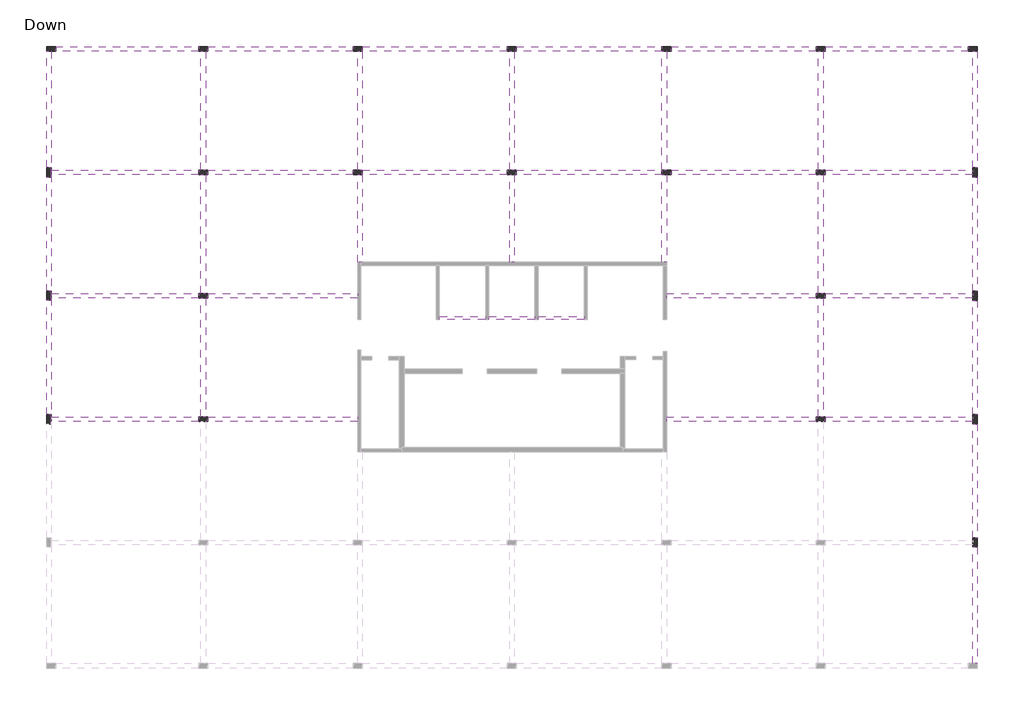
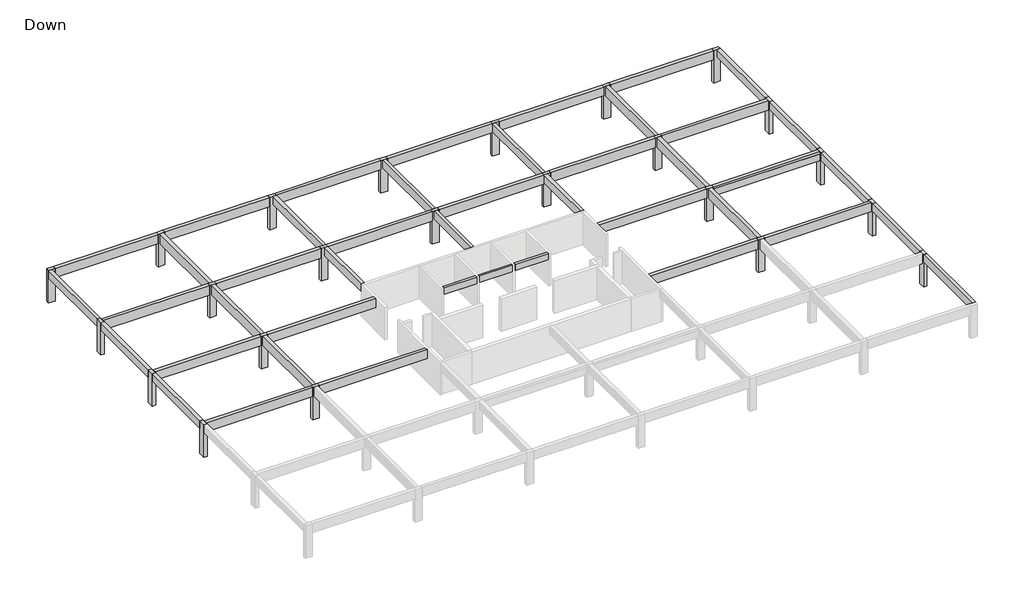
# One storey, part 2 of 2: 43 beams, 23 columns.
"""IFC4 building model written with IfcOpenShell, lengths in millimetres."""

from ifc_helpers import new_model, si_unit, frame, origin, origin_with_axes, place, context, project, spatial, polyline, outline, extrude, faceted_brep, element, save

model = new_model("IFC4")

# Units and contexts
model_context = context("Model", 3, world=origin())
ifc_project = project(units=[si_unit("LENGTHUNIT", "METRE", prefix="MILLI")], contexts=[model_context])

# Site, building, storey
site = spatial("IfcSite", under=ifc_project)
building = spatial("IfcBuilding", under=site)
storey = spatial("IfcBuildingStorey", under=building, Name="Down", Elevation=0.0)

# Beams
placement = place(None, origin())
element("IfcBeam", 1, ObjectType="Concrete Rectengular Beam : 20/60", at=placement, inside=storey, context=model_context, shape_type="SweptSolid", body=[
    extrude(outline(polyline([(-1146.9159577, 7369.5351037), (-1146.9159577, 7569.5351037), (1839.2018335, 7569.5351037), (1839.2018335, 7369.5351037), (-1146.9159577, 7369.5351037)])), frame((0.0, 0.0, 2480.0), z_axis=(0.0, 0.0, 1.0), x_axis=(1.0, 0.0, 0.0)), (0.0, 0.0, 1.0), 600.0),
])
element("IfcBeam", 2, ObjectType="Concrete Rectengular Beam : 20/60", at=placement, inside=storey, context=model_context, shape_type="Brep", body=[
    faceted_brep([(2039.2018335, 7569.5351037, 3080.0), (2039.2018335, 7369.5351037, 3080.0), (5039.2018335, 7369.5351037, 3080.0), (5039.2018335, 7569.5351037, 3080.0), (2039.2018335, 7369.5351037, 2860.0), (2039.2018335, 7369.5351037, 2480.0), (5039.2018335, 7369.5351037, 2480.0), (2039.2018335, 7569.5351037, 2480.0), (5039.2018335, 7569.5351037, 2480.0)], [[[0, 1, 2, 3]], [[1, 4, 5, 6, 2]], [[5, 7, 8, 6]], [[7, 0, 3, 8]], [[1, 0, 7, 5, 4]], [[3, 2, 6, 8]]]),
])
element("IfcBeam", 3, ObjectType="Concrete Rectengular Beam : 20/60", at=placement, inside=storey, context=model_context, shape_type="Brep", body=[
    faceted_brep([(5239.2018335, 7569.5351037, 3080.0), (5239.2018335, 7369.5351037, 3080.0), (8239.2018335, 7369.5351037, 3080.0), (8239.2018335, 7569.5351037, 3080.0), (5239.2018335, 7369.5351037, 2860.0), (5239.2018335, 7369.5351037, 2480.0), (8239.2018335, 7369.5351037, 2480.0), (5239.2018335, 7569.5351037, 2480.0), (8239.2018335, 7569.5351037, 2480.0)], [[[0, 1, 2, 3]], [[1, 4, 5, 6, 2]], [[5, 7, 8, 6]], [[7, 0, 3, 8]], [[1, 0, 7, 5, 4]], [[3, 2, 6, 8]]]),
])
element("IfcBeam", 4, ObjectType="Concrete Rectengular Beam : 30/70", at=placement, inside=storey, context=model_context, shape_type="SweptSolid", body=[
    extrude(outline(polyline([(33698.6447783, 9222.0890048), (33398.6447783, 9222.0890048), (33398.6447783, 16622.0890048), (33698.6447783, 16622.0890048), (33698.6447783, 9222.0890048)])), frame((0.0, 0.0, 2380.0), z_axis=(0.0, 0.0, 1.0), x_axis=(1.0, 0.0, 0.0)), (0.0, 0.0, 1.0), 700.0),
])
element("IfcBeam", 5, ObjectType="Concrete Rectengular Beam : 30/70", at=placement, inside=storey, context=model_context, shape_type="SweptSolid", body=[
    extrude(outline(polyline([(33398.6447783, 8622.0890048), (33698.6447783, 8622.0890048), (33698.6447783, 1224.102585), (33398.6447783, 1224.102585), (33398.6447783, 8622.0890048)])), frame((0.0, 0.0, 2380.0), z_axis=(0.0, 0.0, 1.0), x_axis=(1.0, 0.0, 0.0)), (0.0, 0.0, 1.0), 700.0),
])
element("IfcBeam", 6, ObjectType="Concrete Rectengular Beam : 30/70", at=placement, inside=storey, context=model_context, shape_type="SweptSolid", body=[
    extrude(outline(polyline([(33698.6447783, -6770.4648963), (33398.6447783, -6770.4648963), (33398.6447783, 624.102585), (33698.6447783, 624.102585), (33698.6447783, -6770.4648963)])), frame((0.0, 0.0, 2380.0), z_axis=(0.0, 0.0, 1.0), x_axis=(1.0, 0.0, 0.0)), (0.0, 0.0, 1.0), 700.0),
])
element("IfcBeam", 7, ObjectType="Concrete Rectengular Beam : 30/70", at=placement, inside=storey, context=model_context, shape_type="Brep", body=[
    faceted_brep([(33698.6447783, -7370.4648963, 3080.0), (33398.6447783, -7370.4648963, 3080.0), (33398.6447783, -14918.7716477, 3080.0), (33698.6447783, -14918.7716477, 3080.0), (33398.6447783, -7370.4648963, 2380.0), (33398.6447783, -14918.7716477, 2380.0), (33398.6447783, -14918.7716477, 2860.0), (33698.6447783, -7370.4648963, 2380.0), (33698.6447783, -14918.7716477, 2380.0)], [[[0, 1, 2, 3]], [[1, 4, 5, 6, 2]], [[4, 7, 8, 5]], [[7, 0, 3, 8]], [[1, 0, 7, 4]], [[3, 2, 6, 5, 8]]]),
])
element("IfcBeam", 8, ObjectType="Concrete Rectengular Beam : 30/70", at=placement, inside=storey, context=model_context, shape_type="Brep", body=[
    faceted_brep([(33698.6447783, 24775.4190544, 3080.0), (33398.6447783, 24775.4190544, 3080.0), (33398.6447783, 17222.0890048, 3080.0), (33698.6447783, 17222.0890048, 3080.0), (33398.6447783, 24775.4190544, 2860.0), (33398.6447783, 24775.4190544, 2380.0), (33398.6447783, 17222.0890048, 2380.0), (33698.6447783, 24775.4190544, 2380.0), (33698.6447783, 17222.0890048, 2380.0)], [[[0, 1, 2, 3]], [[1, 4, 5, 6, 2]], [[5, 7, 8, 6]], [[7, 0, 3, 8]], [[1, 0, 7, 5, 4]], [[3, 2, 6, 8]]]),
])
element("IfcBeam", 9, ObjectType="Concrete Rectengular Beam : 30/70", at=placement, inside=storey, context=model_context, shape_type="Brep", body=[
    faceted_brep([(-26299.591421, 9078.7943074, 3080.0), (-26299.591421, 8628.7943074, 3080.0), (-26599.1167382, 8628.7943074, 3080.0), (-26599.1167382, 1224.102585, 3080.0), (-26299.591421, 1224.102585, 3080.0), (-26299.591421, 1074.102585, 3080.0), (-26299.1167382, 1074.102585, 3080.0), (-26299.1167382, 8778.7943074, 3080.0), (-26299.1167382, 9078.7943074, 3080.0), (-26299.1167382, 9078.7943074, 2380.0), (-26299.1167382, 1074.102585, 2860.0), (-26299.1167382, 1074.102585, 2380.0), (-26299.1167382, 8778.7943074, 2380.0), (-26299.591421, 8628.7943074, 2380.0), (-26299.591421, 8778.7943074, 2380.0), (-26299.591421, 9078.7943074, 2380.0), (-26299.591421, 1074.102585, 2380.0), (-26299.591421, 1224.102585, 2380.0), (-26599.1167382, 1224.102585, 2380.0), (-26599.1167382, 8628.7943074, 2380.0)], [[[0, 1, 2, 3, 4, 5, 6, 7, 8]], [[9, 8, 7, 6, 10, 11, 12]], [[13, 14, 15, 9, 12, 11, 16, 17, 18, 19]], [[2, 19, 18, 3]], [[13, 1, 0, 15, 14]], [[1, 13, 19, 2]], [[17, 4, 3, 18]], [[4, 17, 16, 5]], [[8, 9, 15, 0]], [[11, 10, 6, 5, 16]]]),
])
element("IfcBeam", 10, ObjectType="Concrete Rectengular Beam : 30/70", at=placement, inside=storey, context=model_context, shape_type="Brep", body=[
    faceted_brep([(-26299.591421, 17073.0342824, 3080.0), (-26299.591421, 16623.0342824, 3080.0), (-26599.1167382, 16623.0342824, 3080.0), (-26599.1167382, 9228.7943074, 3080.0), (-26299.591421, 9228.7943074, 3080.0), (-26299.591421, 9078.7943074, 3080.0), (-26299.1167382, 9078.7943074, 3080.0), (-26299.1167382, 16773.0342824, 3080.0), (-26299.1167382, 17073.0342824, 3080.0), (-26299.1167382, 9078.7943074, 2860.0), (-26299.1167382, 9078.7943074, 2380.0), (-26299.1167382, 16773.0342824, 2380.0), (-26299.1167382, 17073.0342824, 2380.0), (-26299.591421, 16623.0342824, 2380.0), (-26299.591421, 16773.0342824, 2380.0), (-26299.591421, 17073.0342824, 2380.0), (-26299.591421, 9078.7943074, 2380.0), (-26299.591421, 9228.7943074, 2380.0), (-26599.1167382, 9228.7943074, 2380.0), (-26599.1167382, 16623.0342824, 2380.0)], [[[0, 1, 2, 3, 4, 5, 6, 7, 8]], [[6, 9, 10, 11, 12, 8, 7]], [[13, 14, 15, 12, 11, 10, 16, 17, 18, 19]], [[2, 19, 18, 3]], [[13, 1, 0, 15, 14]], [[1, 13, 19, 2]], [[17, 4, 3, 18]], [[4, 17, 16, 5]], [[10, 9, 6, 5, 16]], [[8, 12, 15, 0]]]),
])
element("IfcBeam", 11, ObjectType="Concrete Rectengular Beam : 30/70", at=placement, inside=storey, context=model_context, shape_type="Brep", body=[
    faceted_brep([(-26299.1167382, 24775.4190544, 3080.0), (-26599.1167382, 24775.4190544, 3080.0), (-26599.1167382, 17223.0342824, 3080.0), (-26299.591421, 17223.0342824, 3080.0), (-26299.591421, 17073.0342824, 3080.0), (-26299.1167382, 17073.0342824, 3080.0), (-26299.1167382, 24775.4190544, 2380.0), (-26299.1167382, 24775.4190544, 2860.0), (-26299.1167382, 17073.0342824, 2860.0), (-26299.1167382, 17073.0342824, 2380.0), (-26599.1167382, 24775.4190544, 2380.0), (-26299.591421, 17073.0342824, 2380.0), (-26299.591421, 17223.0342824, 2380.0), (-26599.1167382, 17223.0342824, 2380.0)], [[[0, 1, 2, 3, 4, 5]], [[6, 7, 0, 5, 8, 9]], [[10, 6, 9, 11, 12, 13]], [[1, 10, 13, 2]], [[1, 0, 7, 6, 10]], [[12, 3, 2, 13]], [[3, 12, 11, 4]], [[9, 8, 5, 4, 11]]]),
])
element("IfcBeam", 12, ObjectType="Concrete Rectengular Beam : 30/75", at=placement, inside=storey, context=model_context, shape_type="Brep", body=[
    faceted_brep([(-6447.328783, 17073.0342824, 3080.0), (-6147.328783, 17073.0342824, 3080.0), (-6147.328783, 24775.4190544, 3080.0), (-6447.328783, 24775.4190544, 3080.0), (-6447.328783, 17073.0342824, 2330.0), (-6447.328783, 17073.0342824, 2860.0), (-6447.328783, 24775.4190544, 2860.0), (-6447.328783, 24775.4190544, 2330.0), (-6147.328783, 17073.0342824, 2330.0), (-6147.328783, 24775.4190544, 2330.0), (-6147.328783, 17073.0342824, 2860.0), (-6147.328783, 24775.4190544, 2860.0)], [[[0, 1, 2, 3]], [[4, 5, 0, 3, 6, 7]], [[8, 4, 7, 9]], [[1, 10, 8, 9, 11, 2]], [[1, 0, 5, 4, 8, 10]], [[3, 2, 11, 9, 7, 6]]]),
])
element("IfcBeam", 13, ObjectType="Concrete Rectengular Beam : 30/75", at=placement, inside=storey, context=model_context, shape_type="Brep", body=[
    faceted_brep([(-6147.328783, 16773.0342824, 3080.0), (-6447.328783, 16773.0342824, 3080.0), (-6447.328783, 11089.5351037, 3080.0), (-6247.328783, 11089.5351037, 3080.0), (-6147.328783, 11089.5351037, 3080.0), (-6447.328783, 16773.0342824, 2860.0), (-6447.328783, 16773.0342824, 2330.0), (-6447.328783, 11089.5351037, 2330.0), (-6147.328783, 16773.0342824, 2330.0), (-6147.328783, 11089.5351037, 2330.0), (-6147.328783, 16773.0342824, 2860.0), (-6147.328783, 11089.5351037, 2860.0)], [[[0, 1, 2, 3, 4]], [[1, 5, 6, 7, 2]], [[6, 8, 9, 7]], [[8, 10, 0, 4, 11, 9]], [[1, 0, 10, 8, 6, 5]], [[2, 7, 9, 11, 4, 3]]]),
])
element("IfcBeam", 14, ObjectType="Concrete Rectengular Beam : 30/75", at=placement, inside=storey, context=model_context, shape_type="Brep", body=[
    faceted_brep([(3389.2018335, 17073.0342824, 3080.0), (3689.2018335, 17073.0342824, 3080.0), (3689.2018335, 24775.4190544, 3080.0), (3389.2018335, 24775.4190544, 3080.0), (3389.2018335, 17073.0342824, 2330.0), (3389.2018335, 17073.0342824, 2860.0), (3389.2018335, 24775.4190544, 2860.0), (3389.2018335, 24775.4190544, 2330.0), (3689.2018335, 17073.0342824, 2330.0), (3689.2018335, 24775.4190544, 2330.0), (3689.2018335, 17073.0342824, 2860.0), (3689.2018335, 24775.4190544, 2860.0)], [[[0, 1, 2, 3]], [[4, 5, 0, 3, 6, 7]], [[8, 4, 7, 9]], [[1, 10, 8, 9, 11, 2]], [[1, 0, 5, 4, 8, 10]], [[3, 2, 11, 9, 7, 6]]]),
])
element("IfcBeam", 15, ObjectType="Concrete Rectengular Beam : 30/75", at=placement, inside=storey, context=model_context, shape_type="Brep", body=[
    faceted_brep([(3689.2018335, 16773.0342824, 3080.0), (3389.2018335, 16773.0342824, 3080.0), (3389.2018335, 11089.5351037, 3080.0), (3689.2018335, 11089.5351037, 3080.0), (3389.2018335, 16773.0342824, 2860.0), (3389.2018335, 16773.0342824, 2330.0), (3389.2018335, 11089.5351037, 2330.0), (3389.2018335, 11089.5351037, 2860.0), (3689.2018335, 16773.0342824, 2330.0), (3689.2018335, 11089.5351037, 2330.0), (3689.2018335, 16773.0342824, 2860.0), (3689.2018335, 11089.5351037, 2860.0)], [[[0, 1, 2, 3]], [[1, 4, 5, 6, 7, 2]], [[5, 8, 9, 6]], [[8, 10, 0, 3, 11, 9]], [[1, 0, 10, 8, 5, 4]], [[3, 2, 7, 6, 9, 11]]]),
])
element("IfcBeam", 16, ObjectType="Concrete Rectengular Beam : 30/75", at=placement, inside=storey, context=model_context, shape_type="Brep", body=[
    faceted_brep([(13257.9839294, 24775.4190544, 3080.0), (13257.9839294, 17073.0342824, 3080.0), (13525.73245, 17073.0342824, 3080.0), (13525.73245, 24775.4190544, 3080.0), (13257.9839294, 24775.4190544, 2860.0), (13257.9839294, 24775.4190544, 2330.0), (13257.9839294, 17073.0342824, 2330.0), (13257.9839294, 17073.0342824, 2860.0), (13557.9839294, 24775.4190544, 2330.0), (13557.9839294, 17073.0342824, 2330.0), (13557.9839294, 24775.4190544, 2860.0), (13557.9839294, 17073.0342824, 2860.0), (13525.73245, 24775.4190544, 2860.0), (13525.73245, 17073.0342824, 2860.0)], [[[0, 1, 2, 3]], [[0, 4, 5, 6, 7, 1]], [[5, 8, 9, 6]], [[9, 8, 10, 11]], [[5, 4, 0, 3, 12, 10, 8]], [[1, 7, 6, 9, 11, 13, 2]], [[12, 13, 11, 10]], [[13, 12, 3, 2]]]),
])
element("IfcBeam", 17, ObjectType="Concrete Rectengular Beam : 30/75", at=placement, inside=storey, context=model_context, shape_type="Brep", body=[
    faceted_brep([(13557.9839294, 16773.0342824, 3080.0), (13257.9839294, 16773.0342824, 3080.0), (13257.9839294, 11089.5351037, 3080.0), (13557.9839294, 11089.5351037, 3080.0), (13257.9839294, 16773.0342824, 2860.0), (13257.9839294, 16773.0342824, 2330.0), (13257.9839294, 11089.5351037, 2330.0), (13257.9839294, 11089.5351037, 2860.0), (13557.9839294, 16773.0342824, 2330.0), (13557.9839294, 11089.5351037, 2330.0), (13557.9839294, 16773.0342824, 2860.0)], [[[0, 1, 2, 3]], [[1, 4, 5, 6, 7, 2]], [[5, 8, 9, 6]], [[8, 10, 0, 3, 9]], [[1, 0, 10, 8, 5, 4]], [[3, 2, 7, 6, 9]]]),
])
element("IfcBeam", 18, ObjectType="Concrete Rectengular Beam : 30/85", at=placement, inside=storey, context=model_context, shape_type="SweptSolid", body=[
    extrude(outline(polyline([(-25999.1167382, 24775.4190544), (-25999.1167382, 25075.4190544), (-16750.7819865, 25075.4190544), (-16750.7819865, 24775.4190544), (-25999.1167382, 24775.4190544)])), frame((0.0, 0.0, 2230.0), z_axis=(0.0, 0.0, 1.0), x_axis=(1.0, 0.0, 0.0)), (0.0, 0.0, 1.0), 850.0),
])
element("IfcBeam", 19, ObjectType="Concrete Rectengular Beam : 30/85", at=placement, inside=storey, context=model_context, shape_type="SweptSolid", body=[
    extrude(outline(polyline([(-16150.7819865, 24775.4190544), (-16150.7819865, 25075.4190544), (-6747.328783, 25075.4190544), (-6747.328783, 24775.4190544), (-16150.7819865, 24775.4190544)])), frame((0.0, 0.0, 2230.0), z_axis=(0.0, 0.0, 1.0), x_axis=(1.0, 0.0, 0.0)), (0.0, 0.0, 1.0), 850.0),
])
element("IfcBeam", 20, ObjectType="Concrete Rectengular Beam : 30/85", at=placement, inside=storey, context=model_context, shape_type="Brep", body=[
    faceted_brep([(-6147.328783, 25075.4190544, 3080.0), (-6147.328783, 24775.4190544, 3080.0), (3239.2018335, 24775.4190544, 3080.0), (3239.2018335, 25075.4190544, 3080.0), (-6147.328783, 24775.4190544, 2860.0), (-6147.328783, 24775.4190544, 2230.0), (3239.2018335, 24775.4190544, 2230.0), (-6147.328783, 25075.4190544, 2230.0), (3239.2018335, 25075.4190544, 2230.0)], [[[0, 1, 2, 3]], [[1, 4, 5, 6, 2]], [[5, 7, 8, 6]], [[7, 0, 3, 8]], [[7, 5, 4, 1, 0]], [[3, 2, 6, 8]]]),
])
element("IfcBeam", 21, ObjectType="Concrete Rectengular Beam : 30/85", at=placement, inside=storey, context=model_context, shape_type="Brep", body=[
    faceted_brep([(13257.9839294, 24775.4190544, 3080.0), (13257.9839294, 25075.4190544, 3080.0), (3839.2018335, 25075.4190544, 3080.0), (3839.2018335, 24775.4190544, 3080.0), (13257.9839294, 24775.4190544, 2230.0), (13257.9839294, 24775.4190544, 2860.0), (3839.2018335, 24775.4190544, 2230.0), (13257.9839294, 25075.4190544, 2230.0), (3839.2018335, 25075.4190544, 2230.0)], [[[0, 1, 2, 3]], [[4, 5, 0, 3, 6]], [[7, 4, 6, 8]], [[1, 7, 8, 2]], [[1, 0, 5, 4, 7]], [[3, 2, 8, 6]]]),
])
element("IfcBeam", 22, ObjectType="Concrete Rectengular Beam : 30/85", at=placement, inside=storey, context=model_context, shape_type="SweptSolid", body=[
    extrude(outline(polyline([(23250.3644839, 25075.4190544), (23250.3644839, 24775.4190544), (13857.9839294, 24775.4190544), (13857.9839294, 25075.4190544), (23250.3644839, 25075.4190544)])), frame((0.0, 0.0, 2230.0), z_axis=(0.0, 0.0, 1.0), x_axis=(1.0, 0.0, 0.0)), (0.0, 0.0, 1.0), 850.0),
])
element("IfcBeam", 23, ObjectType="Concrete Rectengular Beam : 30/85", at=placement, inside=storey, context=model_context, shape_type="SweptSolid", body=[
    extrude(outline(polyline([(23850.3644839, 24775.4190544), (23850.3644839, 25075.4190544), (33098.6447783, 25075.4190544), (33098.6447783, 24775.4190544), (23850.3644839, 24775.4190544)])), frame((0.0, 0.0, 2230.0), z_axis=(0.0, 0.0, 1.0), x_axis=(1.0, 0.0, 0.0)), (0.0, 0.0, 1.0), 850.0),
])
element("IfcBeam", 24, ObjectType="Concrete Rectengular Beam : 30/85", at=placement, inside=storey, context=model_context, shape_type="Brep", body=[
    faceted_brep([(23850.3644839, 1074.102585, 3080.0), (23850.3644839, 774.102585, 3080.0), (33398.6447783, 774.102585, 3080.0), (33398.6447783, 1074.102585, 3080.0), (23850.3644839, 1074.102585, 2230.0), (33398.6447783, 1074.102585, 2860.0), (33398.6447783, 1074.102585, 2230.0), (23850.3644839, 774.102585, 2230.0), (33398.6447783, 774.102585, 2230.0), (33398.6447783, 774.102585, 2860.0)], [[[0, 1, 2, 3]], [[4, 0, 3, 5, 6]], [[7, 4, 6, 8]], [[1, 7, 8, 9, 2]], [[1, 0, 4, 7]], [[3, 2, 9, 8, 6, 5]]]),
])
element("IfcBeam", 25, ObjectType="Concrete Rectengular Beam : 30/85", at=placement, inside=storey, context=model_context, shape_type="Brep", body=[
    faceted_brep([(23250.3644839, 774.102585, 3080.0), (23250.3644839, 1074.102585, 3080.0), (13557.9839294, 1074.102585, 3080.0), (13557.9839294, 774.102585, 3080.0), (23250.3644839, 1074.102585, 2230.0), (13557.9839294, 1074.102585, 2230.0), (13557.9839294, 1074.102585, 2860.0), (23250.3644839, 774.102585, 2230.0), (13557.9839294, 774.102585, 2230.0), (13557.9839294, 774.102585, 2860.0)], [[[0, 1, 2, 3]], [[1, 4, 5, 6, 2]], [[4, 7, 8, 5]], [[7, 0, 3, 9, 8]], [[1, 0, 7, 4]], [[3, 2, 6, 5, 8, 9]]]),
])
element("IfcBeam", 26, ObjectType="Concrete Rectengular Beam : 30/85", at=placement, inside=storey, context=model_context, shape_type="Brep", body=[
    faceted_brep([(33398.6447783, 9072.0890048, 3080.0), (23850.3644839, 9072.0890048, 3080.0), (23850.3644839, 8778.7943074, 3080.0), (33398.6447783, 8778.7943074, 3080.0), (33398.6447783, 9072.0890048, 2860.0), (33398.6447783, 9072.0890048, 2230.0), (23850.3644839, 9072.0890048, 2230.0), (33398.6447783, 8772.0890048, 2230.0), (23850.3644839, 8772.0890048, 2230.0), (33398.6447783, 8772.0890048, 2860.0), (23850.3644839, 8772.0890048, 2860.0), (33398.6447783, 8778.7943074, 2860.0), (23850.3644839, 8778.7943074, 2860.0)], [[[0, 1, 2, 3]], [[0, 4, 5, 6, 1]], [[5, 7, 8, 6]], [[8, 7, 9, 10]], [[5, 4, 0, 3, 11, 9, 7]], [[1, 6, 8, 10, 12, 2]], [[11, 12, 10, 9]], [[12, 11, 3, 2]]]),
])
element("IfcBeam", 27, ObjectType="Concrete Rectengular Beam : 30/85", at=placement, inside=storey, context=model_context, shape_type="Brep", body=[
    faceted_brep([(23250.3644839, 8772.0890048, 3080.0), (23250.3644839, 9072.0890048, 3080.0), (13557.9839294, 9072.0890048, 3080.0), (13557.9839294, 8772.0890048, 3080.0), (23250.3644839, 9072.0890048, 2230.0), (13557.9839294, 9072.0890048, 2230.0), (13557.9839294, 9072.0890048, 2860.0), (23250.3644839, 8772.0890048, 2230.0), (13557.9839294, 8772.0890048, 2230.0), (13557.9839294, 8772.0890048, 2860.0)], [[[0, 1, 2, 3]], [[1, 4, 5, 6, 2]], [[4, 7, 8, 5]], [[7, 0, 3, 9, 8]], [[1, 0, 7, 4]], [[3, 2, 6, 5, 8, 9]]]),
])
element("IfcBeam", 28, ObjectType="Concrete Rectengular Beam : 30/85", at=placement, inside=storey, context=model_context, shape_type="Brep", body=[
    faceted_brep([(-16750.7819865, 8778.7943074, 3080.0), (-16750.7819865, 9078.7943074, 3080.0), (-26299.1167382, 9078.7943074, 3080.0), (-26299.1167382, 8778.7943074, 3080.0), (-26299.591421, 8778.7943074, 2230.0), (-16750.7819865, 8778.7943074, 2230.0), (-26299.1167382, 8778.7943074, 2860.0), (-26299.1167382, 8778.7943074, 2380.0), (-26299.591421, 8778.7943074, 2380.0), (-26299.591421, 9078.7943074, 2230.0), (-16750.7819865, 9078.7943074, 2230.0), (-26299.591421, 9078.7943074, 2380.0), (-26299.1167382, 9078.7943074, 2380.0), (-26299.1167382, 9078.7943074, 2860.0)], [[[0, 1, 2, 3]], [[4, 5, 0, 3, 6, 7, 8]], [[4, 9, 10, 5]], [[10, 9, 11, 12, 13, 2, 1]], [[9, 4, 8, 11]], [[1, 0, 5, 10]], [[12, 7, 6, 3, 2, 13]], [[7, 12, 11, 8]]]),
])
element("IfcBeam", 29, ObjectType="Concrete Rectengular Beam : 30/85", at=placement, inside=storey, context=model_context, shape_type="Brep", body=[
    faceted_brep([(-16150.7819865, 9078.7943074, 3080.0), (-16150.7819865, 8778.7943074, 3080.0), (-6447.328783, 8778.7943074, 3080.0), (-6447.328783, 9078.7943074, 3080.0), (-16150.7819865, 8778.7943074, 2230.0), (-6447.328783, 8778.7943074, 2230.0), (-6447.328783, 8778.7943074, 2860.0), (-16150.7819865, 9078.7943074, 2230.0), (-6447.328783, 9078.7943074, 2230.0), (-6447.328783, 9078.7943074, 2860.0)], [[[0, 1, 2, 3]], [[1, 4, 5, 6, 2]], [[4, 7, 8, 5]], [[7, 0, 3, 9, 8]], [[1, 0, 7, 4]], [[3, 2, 6, 5, 8, 9]]]),
])
element("IfcBeam", 30, ObjectType="Concrete Rectengular Beam : 30/85", at=placement, inside=storey, context=model_context, shape_type="Brep", body=[
    faceted_brep([(-16750.7819865, 774.102585, 3080.0), (-16750.7819865, 1074.102585, 3080.0), (-26299.1167382, 1074.102585, 3080.0), (-26299.1167382, 774.102585, 3080.0), (-26299.591421, 774.102585, 2230.0), (-16750.7819865, 774.102585, 2230.0), (-26299.1167382, 774.102585, 2860.0), (-26299.1167382, 774.102585, 2380.0), (-26299.591421, 774.102585, 2380.0), (-26299.591421, 1074.102585, 2230.0), (-16750.7819865, 1074.102585, 2230.0), (-26299.591421, 1074.102585, 2380.0), (-26299.1167382, 1074.102585, 2380.0), (-26299.1167382, 1074.102585, 2860.0)], [[[0, 1, 2, 3]], [[4, 5, 0, 3, 6, 7, 8]], [[4, 9, 10, 5]], [[10, 9, 11, 12, 13, 2, 1]], [[9, 4, 8, 11]], [[1, 0, 5, 10]], [[12, 7, 6, 3, 2, 13]], [[7, 12, 11, 8]]]),
])
element("IfcBeam", 31, ObjectType="Concrete Rectengular Beam : 30/85", at=placement, inside=storey, context=model_context, shape_type="Brep", body=[
    faceted_brep([(-16150.7819865, 1074.102585, 3080.0), (-16150.7819865, 774.102585, 3080.0), (-6447.328783, 774.102585, 3080.0), (-6447.328783, 1074.102585, 3080.0), (-16150.7819865, 774.102585, 2230.0), (-6447.328783, 774.102585, 2230.0), (-6447.328783, 774.102585, 2860.0), (-16150.7819865, 1074.102585, 2230.0), (-6447.328783, 1074.102585, 2230.0), (-6447.328783, 1074.102585, 2860.0)], [[[0, 1, 2, 3]], [[1, 4, 5, 6, 2]], [[4, 7, 8, 5]], [[7, 0, 3, 9, 8]], [[1, 0, 7, 4]], [[3, 2, 6, 5, 8, 9]]]),
])
element("IfcBeam", 32, ObjectType="Concrete Rectengular Beam : 30/90", at=placement, inside=storey, context=model_context, shape_type="Brep", body=[
    faceted_brep([(23850.3644839, 17073.0342824, 3080.0), (23850.3644839, 16773.0342824, 3080.0), (33398.6447783, 16773.0342824, 3080.0), (33398.6447783, 17073.0342824, 3080.0), (23850.3644839, 17073.0342824, 2180.0), (33398.6447783, 17073.0342824, 2860.0), (33398.6447783, 17073.0342824, 2180.0), (23850.3644839, 16773.0342824, 2180.0), (33398.6447783, 16773.0342824, 2180.0), (33398.6447783, 16773.0342824, 2860.0)], [[[0, 1, 2, 3]], [[4, 0, 3, 5, 6]], [[7, 4, 6, 8]], [[1, 7, 8, 9, 2]], [[1, 0, 4, 7]], [[3, 2, 9, 8, 6, 5]]]),
])
element("IfcBeam", 33, ObjectType="Concrete Rectengular Beam : 30/90", at=placement, inside=storey, context=model_context, shape_type="SweptSolid", body=[
    extrude(outline(polyline([(23250.3644839, 17073.0342824), (23250.3644839, 16773.0342824), (13857.9839294, 16773.0342824), (13857.9839294, 17073.0342824), (23250.3644839, 17073.0342824)])), frame((0.0, 0.0, 2180.0), z_axis=(0.0, 0.0, 1.0), x_axis=(1.0, 0.0, 0.0)), (0.0, 0.0, 1.0), 900.0),
])
element("IfcBeam", 34, ObjectType="Concrete Rectengular Beam : 30/90", at=placement, inside=storey, context=model_context, shape_type="Brep", body=[
    faceted_brep([(13257.9839294, 16773.0342824, 3080.0), (13257.9839294, 17073.0342824, 3080.0), (3839.2018335, 17073.0342824, 3080.0), (3839.2018335, 16773.0342824, 3080.0), (13257.9839294, 17073.0342824, 2860.0), (13257.9839294, 17073.0342824, 2180.0), (3839.2018335, 17073.0342824, 2180.0), (13257.9839294, 16773.0342824, 2180.0), (3839.2018335, 16773.0342824, 2180.0), (13257.9839294, 16773.0342824, 2860.0)], [[[0, 1, 2, 3]], [[1, 4, 5, 6, 2]], [[5, 7, 8, 6]], [[7, 9, 0, 3, 8]], [[7, 5, 4, 1, 0, 9]], [[3, 2, 6, 8]]]),
])
element("IfcBeam", 35, ObjectType="Concrete Rectengular Beam : 30/90", at=placement, inside=storey, context=model_context, shape_type="Brep", body=[
    faceted_brep([(-6147.328783, 17073.0342824, 3080.0), (-6147.328783, 16773.0342824, 3080.0), (3239.2018335, 16773.0342824, 3080.0), (3239.2018335, 17073.0342824, 3080.0), (-6147.328783, 17073.0342824, 2180.0), (-6147.328783, 17073.0342824, 2860.0), (3239.2018335, 17073.0342824, 2180.0), (-6147.328783, 16773.0342824, 2180.0), (3239.2018335, 16773.0342824, 2180.0), (-6147.328783, 16773.0342824, 2860.0)], [[[0, 1, 2, 3]], [[4, 5, 0, 3, 6]], [[7, 4, 6, 8]], [[1, 9, 7, 8, 2]], [[1, 0, 5, 4, 7, 9]], [[3, 2, 8, 6]]]),
])
element("IfcBeam", 36, ObjectType="Concrete Rectengular Beam : 30/90", at=placement, inside=storey, context=model_context, shape_type="SweptSolid", body=[
    extrude(outline(polyline([(-16150.7819865, 16773.0342824), (-16150.7819865, 17073.0342824), (-6747.328783, 17073.0342824), (-6747.328783, 16773.0342824), (-16150.7819865, 16773.0342824)])), frame((0.0, 0.0, 2180.0), z_axis=(0.0, 0.0, 1.0), x_axis=(1.0, 0.0, 0.0)), (0.0, 0.0, 1.0), 900.0),
])
element("IfcBeam", 37, ObjectType="Concrete Rectengular Beam : 30/90", at=placement, inside=storey, context=model_context, shape_type="Brep", body=[
    faceted_brep([(-16750.7819865, 16773.0342824, 3080.0), (-16750.7819865, 17073.0342824, 3080.0), (-26299.1167382, 17073.0342824, 3080.0), (-26299.1167382, 16773.0342824, 3080.0), (-16750.7819865, 17073.0342824, 2180.0), (-26299.591421, 17073.0342824, 2180.0), (-26299.591421, 17073.0342824, 2380.0), (-26299.1167382, 17073.0342824, 2380.0), (-26299.1167382, 17073.0342824, 2860.0), (-26299.591421, 16773.0342824, 2180.0), (-16750.7819865, 16773.0342824, 2180.0), (-26299.1167382, 16773.0342824, 2860.0), (-26299.1167382, 16773.0342824, 2380.0), (-26299.591421, 16773.0342824, 2380.0)], [[[0, 1, 2, 3]], [[4, 5, 6, 7, 8, 2, 1]], [[9, 5, 4, 10]], [[9, 10, 0, 3, 11, 12, 13]], [[5, 9, 13, 6]], [[1, 0, 10, 4]], [[7, 12, 11, 3, 2, 8]], [[12, 7, 6, 13]]]),
])
element("IfcBeam", 38, ObjectType="Concrete Rectengular Beam : 30/90", at=placement, inside=storey, context=model_context, shape_type="Brep", body=[
    faceted_brep([(-16300.7819865, 24775.4190544, 3080.0), (-16600.7819865, 24775.4190544, 3080.0), (-16600.7819865, 17073.0342824, 3080.0), (-16300.7819865, 17073.0342824, 3080.0), (-16600.7819865, 24775.4190544, 2860.0), (-16600.7819865, 24775.4190544, 2180.0), (-16600.7819865, 17073.0342824, 2180.0), (-16600.7819865, 17073.0342824, 2860.0), (-16300.7819865, 24775.4190544, 2180.0), (-16300.7819865, 17073.0342824, 2180.0), (-16300.7819865, 24775.4190544, 2860.0), (-16300.7819865, 17073.0342824, 2860.0)], [[[0, 1, 2, 3]], [[1, 4, 5, 6, 7, 2]], [[5, 8, 9, 6]], [[8, 10, 0, 3, 11, 9]], [[1, 0, 10, 8, 5, 4]], [[2, 7, 6, 9, 11, 3]]]),
])
element("IfcBeam", 39, ObjectType="Concrete Rectengular Beam : 30/90", at=placement, inside=storey, context=model_context, shape_type="Brep", body=[
    faceted_brep([(-16300.7819865, 16773.0342824, 3080.0), (-16600.7819865, 16773.0342824, 3080.0), (-16600.7819865, 9078.7943074, 3080.0), (-16300.7819865, 9078.7943074, 3080.0), (-16600.7819865, 16773.0342824, 2860.0), (-16600.7819865, 16773.0342824, 2180.0), (-16600.7819865, 9078.7943074, 2180.0), (-16600.7819865, 9078.7943074, 2860.0), (-16300.7819865, 16773.0342824, 2180.0), (-16300.7819865, 9078.7943074, 2180.0), (-16300.7819865, 16773.0342824, 2860.0), (-16300.7819865, 9078.7943074, 2860.0)], [[[0, 1, 2, 3]], [[1, 4, 5, 6, 7, 2]], [[5, 8, 9, 6]], [[8, 10, 0, 3, 11, 9]], [[0, 10, 8, 5, 4, 1]], [[3, 2, 7, 6, 9, 11]]]),
])
element("IfcBeam", 40, ObjectType="Concrete Rectengular Beam : 30/90", at=placement, inside=storey, context=model_context, shape_type="Brep", body=[
    faceted_brep([(-16300.7819865, 8778.7943074, 3080.0), (-16600.7819865, 8778.7943074, 3080.0), (-16600.7819865, 1074.102585, 3080.0), (-16300.7819865, 1074.102585, 3080.0), (-16600.7819865, 8778.7943074, 2860.0), (-16600.7819865, 8778.7943074, 2180.0), (-16600.7819865, 1074.102585, 2180.0), (-16600.7819865, 1074.102585, 2860.0), (-16300.7819865, 8778.7943074, 2180.0), (-16300.7819865, 1074.102585, 2180.0), (-16300.7819865, 8778.7943074, 2860.0), (-16300.7819865, 1074.102585, 2860.0)], [[[0, 1, 2, 3]], [[1, 4, 5, 6, 7, 2]], [[5, 8, 9, 6]], [[8, 10, 0, 3, 11, 9]], [[8, 5, 4, 1, 0, 10]], [[3, 2, 7, 6, 9, 11]]]),
])
element("IfcBeam", 41, ObjectType="Concrete Rectengular Beam : 30/90", at=placement, inside=storey, context=model_context, shape_type="Brep", body=[
    faceted_brep([(23700.3644839, 24775.4190544, 3080.0), (23400.3644839, 24775.4190544, 3080.0), (23400.3644839, 17073.0342824, 3080.0), (23700.3644839, 17073.0342824, 3080.0), (23400.3644839, 24775.4190544, 2860.0), (23400.3644839, 24775.4190544, 2180.0), (23400.3644839, 17073.0342824, 2180.0), (23400.3644839, 17073.0342824, 2860.0), (23700.3644839, 24775.4190544, 2180.0), (23700.3644839, 17073.0342824, 2180.0), (23700.3644839, 24775.4190544, 2860.0), (23700.3644839, 17073.0342824, 2860.0)], [[[0, 1, 2, 3]], [[1, 4, 5, 6, 7, 2]], [[5, 8, 9, 6]], [[8, 10, 0, 3, 11, 9]], [[1, 0, 10, 8, 5, 4]], [[2, 7, 6, 9, 11, 3]]]),
])
element("IfcBeam", 42, ObjectType="Concrete Rectengular Beam : 30/90", at=placement, inside=storey, context=model_context, shape_type="Brep", body=[
    faceted_brep([(23400.3644839, 9072.0890048, 3080.0), (23700.3644839, 9072.0890048, 3080.0), (23700.3644839, 16773.0342824, 3080.0), (23400.3644839, 16773.0342824, 3080.0), (23400.3644839, 9072.0890048, 2180.0), (23400.3644839, 9072.0890048, 2860.0), (23400.3644839, 16773.0342824, 2860.0), (23400.3644839, 16773.0342824, 2180.0), (23700.3644839, 9072.0890048, 2180.0), (23700.3644839, 16773.0342824, 2180.0), (23700.3644839, 9072.0890048, 2860.0), (23700.3644839, 16773.0342824, 2860.0)], [[[0, 1, 2, 3]], [[4, 5, 0, 3, 6, 7]], [[8, 4, 7, 9]], [[1, 10, 8, 9, 11, 2]], [[1, 0, 5, 4, 8, 10]], [[2, 11, 9, 7, 6, 3]]]),
])
element("IfcBeam", 43, ObjectType="Concrete Rectengular Beam : 30/90", at=placement, inside=storey, context=model_context, shape_type="Brep", body=[
    faceted_brep([(23700.3644839, 8772.0890048, 3080.0), (23400.3644839, 8772.0890048, 3080.0), (23400.3644839, 1074.102585, 3080.0), (23700.3644839, 1074.102585, 3080.0), (23400.3644839, 8772.0890048, 2860.0), (23400.3644839, 8772.0890048, 2180.0), (23400.3644839, 1074.102585, 2180.0), (23400.3644839, 1074.102585, 2860.0), (23700.3644839, 8772.0890048, 2180.0), (23700.3644839, 1074.102585, 2180.0), (23700.3644839, 8772.0890048, 2860.0), (23700.3644839, 1074.102585, 2860.0)], [[[0, 1, 2, 3]], [[1, 4, 5, 6, 7, 2]], [[5, 8, 9, 6]], [[8, 10, 0, 3, 11, 9]], [[5, 4, 1, 0, 10, 8]], [[3, 2, 7, 6, 9, 11]]]),
])

# Columns
element("IfcColumn", 44, ObjectType="Concrete Rectengular Column : 30/60", at=placement, inside=storey, context=model_context, shape_type="Brep", body=[
    faceted_brep([(33398.6447783, 8622.0890048, 0.0), (33398.6447783, 9222.0890048, 0.0), (33698.6447783, 9222.0890048, 0.0), (33698.6447783, 8622.0890048, 0.0), (33398.6447783, 8622.0890048, 3080.0), (33398.6447783, 8778.7943074, 3080.0), (33398.6447783, 9072.0890048, 3080.0), (33398.6447783, 9222.0890048, 3080.0), (33698.6447783, 9222.0890048, 3080.0), (33698.6447783, 8622.0890048, 3080.0)], [[[0, 1, 2, 3]], [[4, 5, 6, 7, 1, 0]], [[7, 8, 2, 1]], [[8, 9, 3, 2]], [[9, 4, 0, 3]], [[4, 9, 8, 7, 6, 5]]]),
])
element("IfcColumn", 45, ObjectType="Concrete Rectengular Column : 30/60", at=placement, inside=storey, context=model_context, shape_type="Brep", body=[
    faceted_brep([(33698.6447783, -6770.4648963, 0.0), (33698.6447783, -7370.4648963, 0.0), (33398.6447783, -7370.4648963, 0.0), (33398.6447783, -6770.4648963, 0.0), (33698.6447783, -6770.4648963, 3080.0), (33698.6447783, -7370.4648963, 3080.0), (33398.6447783, -7370.4648963, 3080.0), (33398.6447783, -7220.4648963, 3080.0), (33398.6447783, -6920.4648963, 3080.0), (33398.6447783, -6770.4648963, 3080.0)], [[[0, 1, 2, 3]], [[4, 5, 1, 0]], [[5, 6, 2, 1]], [[6, 7, 8, 9, 3, 2]], [[9, 4, 0, 3]], [[4, 9, 8, 7, 6, 5]]]),
])
element("IfcColumn", 46, ObjectType="Concrete Rectengular Column : 30/60", at=placement, inside=storey, context=model_context, shape_type="Brep", body=[
    faceted_brep([(23850.3644839, 8772.0890048, 0.0), (23250.3644839, 8772.0890048, 0.0), (23250.3644839, 9072.0890048, 0.0), (23850.3644839, 9072.0890048, 0.0), (23850.3644839, 8772.0890048, 3080.0), (23700.3644839, 8772.0890048, 3080.0), (23400.3644839, 8772.0890048, 3080.0), (23250.3644839, 8772.0890048, 3080.0), (23850.3644839, 8772.0890048, 2860.0), (23250.3644839, 9072.0890048, 3080.0), (23400.3644839, 9072.0890048, 3080.0), (23700.3644839, 9072.0890048, 3080.0), (23850.3644839, 9072.0890048, 3080.0), (23850.3644839, 8778.7943074, 3080.0)], [[[0, 1, 2, 3]], [[4, 5, 6, 7, 1, 0, 8]], [[7, 9, 2, 1]], [[9, 10, 11, 12, 3, 2]], [[12, 13, 4, 8, 0, 3]], [[4, 13, 12, 11, 10, 9, 7, 6, 5]]]),
])
element("IfcColumn", 47, ObjectType="Concrete Rectengular Column : 30/60", at=placement, inside=storey, context=model_context, shape_type="Brep", body=[
    faceted_brep([(23850.3644839, 24775.4190544, 0.0), (23250.3644839, 24775.4190544, 0.0), (23250.3644839, 25075.4190544, 0.0), (23850.3644839, 25075.4190544, 0.0), (23850.3644839, 24775.4190544, 3080.0), (23700.3644839, 24775.4190544, 3080.0), (23400.3644839, 24775.4190544, 3080.0), (23250.3644839, 24775.4190544, 3080.0), (23250.3644839, 25075.4190544, 3080.0), (23850.3644839, 25075.4190544, 3080.0)], [[[0, 1, 2, 3]], [[4, 5, 6, 7, 1, 0]], [[7, 8, 2, 1]], [[8, 9, 3, 2]], [[9, 4, 0, 3]], [[4, 9, 8, 7, 6, 5]]]),
])
element("IfcColumn", 48, ObjectType="Concrete Rectengular Column : 30/60", at=placement, inside=storey, context=model_context, shape_type="Brep", body=[
    faceted_brep([(23850.3644839, 16773.0342824, 0.0), (23250.3644839, 16773.0342824, 0.0), (23250.3644839, 17073.0342824, 0.0), (23850.3644839, 17073.0342824, 0.0), (23850.3644839, 16773.0342824, 3080.0), (23700.3644839, 16773.0342824, 3080.0), (23400.3644839, 16773.0342824, 3080.0), (23250.3644839, 16773.0342824, 3080.0), (23250.3644839, 17073.0342824, 3080.0), (23400.3644839, 17073.0342824, 3080.0), (23700.3644839, 17073.0342824, 3080.0), (23850.3644839, 17073.0342824, 3080.0)], [[[0, 1, 2, 3]], [[4, 5, 6, 7, 1, 0]], [[7, 8, 2, 1]], [[8, 9, 10, 11, 3, 2]], [[11, 4, 0, 3]], [[4, 11, 10, 9, 8, 7, 6, 5]]]),
])
element("IfcColumn", 49, ObjectType="Concrete Rectengular Column : 30/60", at=placement, inside=storey, context=model_context, shape_type="Brep", body=[
    faceted_brep([(-25999.1167382, 24775.4190544, 0.0), (-26599.1167382, 24775.4190544, 0.0), (-26599.1167382, 25075.4190544, 0.0), (-25999.1167382, 25075.4190544, 0.0), (-25999.1167382, 24775.4190544, 3080.0), (-26299.1167382, 24775.4190544, 3080.0), (-26599.1167382, 24775.4190544, 3080.0), (-26599.1167382, 25075.4190544, 3080.0), (-25999.1167382, 25075.4190544, 3080.0)], [[[0, 1, 2, 3]], [[4, 5, 6, 1, 0]], [[6, 7, 2, 1]], [[7, 8, 3, 2]], [[8, 4, 0, 3]], [[4, 8, 7, 6, 5]]]),
])
element("IfcColumn", 50, ObjectType="Concrete Rectengular Column : 30/60", at=placement, inside=storey, context=model_context, shape_type="Brep", body=[
    faceted_brep([(-16150.7819865, 24775.4190544, 0.0), (-16750.7819865, 24775.4190544, 0.0), (-16750.7819865, 25075.4190544, 0.0), (-16150.7819865, 25075.4190544, 0.0), (-16150.7819865, 24775.4190544, 3080.0), (-16300.7819865, 24775.4190544, 3080.0), (-16600.7819865, 24775.4190544, 3080.0), (-16750.7819865, 24775.4190544, 3080.0), (-16750.7819865, 25075.4190544, 3080.0), (-16150.7819865, 25075.4190544, 3080.0)], [[[0, 1, 2, 3]], [[4, 5, 6, 7, 1, 0]], [[7, 8, 2, 1]], [[8, 9, 3, 2]], [[9, 4, 0, 3]], [[4, 9, 8, 7, 6, 5]]]),
])
element("IfcColumn", 51, ObjectType="Concrete Rectengular Column : 30/60", at=placement, inside=storey, context=model_context, shape_type="SweptSolid", body=[
    extrude(outline(polyline([(-26599.591421, 16623.0342824), (-26599.591421, 17223.0342824), (-26299.591421, 17223.0342824), (-26299.591421, 16623.0342824), (-26599.591421, 16623.0342824)])), origin_with_axes(), (0.0, 0.0, 1.0), 3080.0),
])
element("IfcColumn", 52, ObjectType="Concrete Rectengular Column : 30/60", at=placement, inside=storey, context=model_context, shape_type="Brep", body=[
    faceted_brep([(-16150.7819865, 16773.0342824, 0.0), (-16750.7819865, 16773.0342824, 0.0), (-16750.7819865, 17073.0342824, 0.0), (-16150.7819865, 17073.0342824, 0.0), (-16150.7819865, 16773.0342824, 3080.0), (-16300.7819865, 16773.0342824, 3080.0), (-16600.7819865, 16773.0342824, 3080.0), (-16750.7819865, 16773.0342824, 3080.0), (-16750.7819865, 17073.0342824, 3080.0), (-16600.7819865, 17073.0342824, 3080.0), (-16300.7819865, 17073.0342824, 3080.0), (-16150.7819865, 17073.0342824, 3080.0)], [[[0, 1, 2, 3]], [[4, 5, 6, 7, 1, 0]], [[7, 8, 2, 1]], [[8, 9, 10, 11, 3, 2]], [[11, 4, 0, 3]], [[4, 11, 10, 9, 8, 7, 6, 5]]]),
])
element("IfcColumn", 53, ObjectType="Concrete Rectengular Column : 30/60", at=placement, inside=storey, context=model_context, shape_type="SweptSolid", body=[
    extrude(outline(polyline([(-26599.591421, 8628.7943074), (-26599.591421, 9228.7943074), (-26299.591421, 9228.7943074), (-26299.591421, 8628.7943074), (-26599.591421, 8628.7943074)])), origin_with_axes(), (0.0, 0.0, 1.0), 3080.0),
])
element("IfcColumn", 54, ObjectType="Concrete Rectengular Column : 30/60", at=placement, inside=storey, context=model_context, shape_type="Brep", body=[
    faceted_brep([(-16150.7819865, 8778.7943074, 0.0), (-16750.7819865, 8778.7943074, 0.0), (-16750.7819865, 9078.7943074, 0.0), (-16150.7819865, 9078.7943074, 0.0), (-16150.7819865, 8778.7943074, 3080.0), (-16300.7819865, 8778.7943074, 3080.0), (-16600.7819865, 8778.7943074, 3080.0), (-16750.7819865, 8778.7943074, 3080.0), (-16750.7819865, 9078.7943074, 3080.0), (-16600.7819865, 9078.7943074, 3080.0), (-16300.7819865, 9078.7943074, 3080.0), (-16150.7819865, 9078.7943074, 3080.0)], [[[0, 1, 2, 3]], [[4, 5, 6, 7, 1, 0]], [[7, 8, 2, 1]], [[8, 9, 10, 11, 3, 2]], [[11, 4, 0, 3]], [[4, 11, 10, 9, 8, 7, 6, 5]]]),
])
element("IfcColumn", 55, ObjectType="Concrete Rectengular Column : 30/60", at=placement, inside=storey, context=model_context, shape_type="Brep", body=[
    faceted_brep([(33098.6447783, 25075.4190544, 0.0), (33698.6447783, 25075.4190544, 0.0), (33698.6447783, 24775.4190544, 0.0), (33098.6447783, 24775.4190544, 0.0), (33098.6447783, 25075.4190544, 3080.0), (33698.6447783, 25075.4190544, 3080.0), (33698.6447783, 24775.4190544, 3080.0), (33398.6447783, 24775.4190544, 3080.0), (33098.6447783, 24775.4190544, 3080.0)], [[[0, 1, 2, 3]], [[4, 5, 1, 0]], [[5, 6, 2, 1]], [[6, 7, 8, 3, 2]], [[8, 4, 0, 3]], [[4, 8, 7, 6, 5]]]),
])
element("IfcColumn", 56, ObjectType="Concrete Rectengular Column : 30/60", at=placement, inside=storey, context=model_context, shape_type="Brep", body=[
    faceted_brep([(33398.6447783, 16622.0890048, 0.0), (33398.6447783, 17222.0890048, 0.0), (33698.6447783, 17222.0890048, 0.0), (33698.6447783, 16622.0890048, 0.0), (33398.6447783, 16622.0890048, 3080.0), (33398.6447783, 16773.0342824, 3080.0), (33398.6447783, 17073.0342824, 3080.0), (33398.6447783, 17222.0890048, 3080.0), (33698.6447783, 17222.0890048, 3080.0), (33698.6447783, 16622.0890048, 3080.0)], [[[0, 1, 2, 3]], [[4, 5, 6, 7, 1, 0]], [[7, 8, 2, 1]], [[8, 9, 3, 2]], [[9, 4, 0, 3]], [[4, 9, 8, 7, 6, 5]]]),
])
element("IfcColumn", 57, ObjectType="Concrete Rectengular Column : 30/60", at=placement, inside=storey, context=model_context, shape_type="Brep", body=[
    faceted_brep([(13257.9839294, 25075.4190544, 0.0), (13857.9839294, 25075.4190544, 0.0), (13857.9839294, 24775.4190544, 0.0), (13257.9839294, 24775.4190544, 0.0), (13257.9839294, 25075.4190544, 3080.0), (13857.9839294, 25075.4190544, 3080.0), (13857.9839294, 24775.4190544, 3080.0), (13525.73245, 24775.4190544, 3080.0), (13257.9839294, 24775.4190544, 3080.0)], [[[0, 1, 2, 3]], [[4, 5, 1, 0]], [[5, 6, 2, 1]], [[6, 7, 8, 3, 2]], [[8, 4, 0, 3]], [[4, 8, 7, 6, 5]]]),
])
element("IfcColumn", 58, ObjectType="Concrete Rectengular Column : 30/60", at=placement, inside=storey, context=model_context, shape_type="Brep", body=[
    faceted_brep([(13257.9839294, 17073.0342824, 0.0), (13857.9839294, 17073.0342824, 0.0), (13857.9839294, 16773.0342824, 0.0), (13257.9839294, 16773.0342824, 0.0), (13257.9839294, 17073.0342824, 3080.0), (13525.73245, 17073.0342824, 3080.0), (13857.9839294, 17073.0342824, 3080.0), (13857.9839294, 16773.0342824, 3080.0), (13557.9839294, 16773.0342824, 3080.0), (13257.9839294, 16773.0342824, 3080.0)], [[[0, 1, 2, 3]], [[4, 5, 6, 1, 0]], [[6, 7, 2, 1]], [[7, 8, 9, 3, 2]], [[9, 4, 0, 3]], [[4, 9, 8, 7, 6, 5]]]),
])
element("IfcColumn", 59, ObjectType="Concrete Rectengular Column : 30/60", at=placement, inside=storey, context=model_context, shape_type="Brep", body=[
    faceted_brep([(23250.3644839, 1074.102585, 0.0), (23850.3644839, 1074.102585, 0.0), (23850.3644839, 774.102585, 0.0), (23250.3644839, 774.102585, 0.0), (23250.3644839, 1074.102585, 3080.0), (23400.3644839, 1074.102585, 3080.0), (23700.3644839, 1074.102585, 3080.0), (23850.3644839, 1074.102585, 3080.0), (23850.3644839, 774.102585, 3080.0), (23700.3644839, 774.102585, 3080.0), (23400.3644839, 774.102585, 3080.0), (23250.3644839, 774.102585, 3080.0)], [[[0, 1, 2, 3]], [[4, 5, 6, 7, 1, 0]], [[7, 8, 2, 1]], [[8, 9, 10, 11, 3, 2]], [[11, 4, 0, 3]], [[4, 11, 10, 9, 8, 7, 6, 5]]]),
])
element("IfcColumn", 60, ObjectType="Concrete Rectengular Column : 30/60", at=placement, inside=storey, context=model_context, shape_type="SweptSolid", body=[
    extrude(outline(polyline([(-26599.591421, 624.102585), (-26599.591421, 1224.102585), (-26299.591421, 1224.102585), (-26299.591421, 624.102585), (-26599.591421, 624.102585)])), origin_with_axes(), (0.0, 0.0, 1.0), 3080.0),
])
element("IfcColumn", 61, ObjectType="Concrete Rectengular Column : 30/60", at=placement, inside=storey, context=model_context, shape_type="Brep", body=[
    faceted_brep([(-16150.7819865, 774.102585, 0.0), (-16750.7819865, 774.102585, 0.0), (-16750.7819865, 1074.102585, 0.0), (-16150.7819865, 1074.102585, 0.0), (-16150.7819865, 774.102585, 3080.0), (-16300.7819865, 774.102585, 3080.0), (-16600.7819865, 774.102585, 3080.0), (-16750.7819865, 774.102585, 3080.0), (-16750.7819865, 1074.102585, 3080.0), (-16600.7819865, 1074.102585, 3080.0), (-16300.7819865, 1074.102585, 3080.0), (-16150.7819865, 1074.102585, 3080.0)], [[[0, 1, 2, 3]], [[4, 5, 6, 7, 1, 0]], [[7, 8, 2, 1]], [[8, 9, 10, 11, 3, 2]], [[11, 4, 0, 3]], [[4, 11, 10, 9, 8, 7, 6, 5]]]),
])
element("IfcColumn", 62, ObjectType="Concrete Rectengular Column : 30/60", at=placement, inside=storey, context=model_context, shape_type="Brep", body=[
    faceted_brep([(-6147.328783, 16773.0342824, 0.0), (-6747.328783, 16773.0342824, 0.0), (-6747.328783, 17073.0342824, 0.0), (-6147.328783, 17073.0342824, 0.0), (-6147.328783, 16773.0342824, 3080.0), (-6447.328783, 16773.0342824, 3080.0), (-6747.328783, 16773.0342824, 3080.0), (-6747.328783, 17073.0342824, 3080.0), (-6447.328783, 17073.0342824, 3080.0), (-6147.328783, 17073.0342824, 3080.0)], [[[0, 1, 2, 3]], [[4, 5, 6, 1, 0]], [[6, 7, 2, 1]], [[7, 8, 9, 3, 2]], [[9, 4, 0, 3]], [[4, 9, 8, 7, 6, 5]]]),
])
element("IfcColumn", 63, ObjectType="Concrete Rectengular Column : 30/60", at=placement, inside=storey, context=model_context, shape_type="Brep", body=[
    faceted_brep([(-6147.328783, 24775.4190544, 0.0), (-6747.328783, 24775.4190544, 0.0), (-6747.328783, 25075.4190544, 0.0), (-6147.328783, 25075.4190544, 0.0), (-6147.328783, 24775.4190544, 3080.0), (-6447.328783, 24775.4190544, 3080.0), (-6747.328783, 24775.4190544, 3080.0), (-6747.328783, 25075.4190544, 3080.0), (-6147.328783, 25075.4190544, 3080.0)], [[[0, 1, 2, 3]], [[4, 5, 6, 1, 0]], [[6, 7, 2, 1]], [[7, 8, 3, 2]], [[8, 4, 0, 3]], [[4, 8, 7, 6, 5]]]),
])
element("IfcColumn", 64, ObjectType="Concrete Rectengular Column : 30/60", at=placement, inside=storey, context=model_context, shape_type="Brep", body=[
    faceted_brep([(3839.2018335, 16773.0342824, 0.0), (3239.2018335, 16773.0342824, 0.0), (3239.2018335, 17073.0342824, 0.0), (3839.2018335, 17073.0342824, 0.0), (3839.2018335, 16773.0342824, 3080.0), (3689.2018335, 16773.0342824, 3080.0), (3389.2018335, 16773.0342824, 3080.0), (3239.2018335, 16773.0342824, 3080.0), (3239.2018335, 17073.0342824, 3080.0), (3389.2018335, 17073.0342824, 3080.0), (3689.2018335, 17073.0342824, 3080.0), (3839.2018335, 17073.0342824, 3080.0)], [[[0, 1, 2, 3]], [[4, 5, 6, 7, 1, 0]], [[7, 8, 2, 1]], [[8, 9, 10, 11, 3, 2]], [[11, 4, 0, 3]], [[4, 11, 10, 9, 8, 7, 6, 5]]]),
])
element("IfcColumn", 65, ObjectType="Concrete Rectengular Column : 30/60", at=placement, inside=storey, context=model_context, shape_type="Brep", body=[
    faceted_brep([(33698.6447783, 1224.102585, 0.0), (33698.6447783, 624.102585, 0.0), (33398.6447783, 624.102585, 0.0), (33398.6447783, 1224.102585, 0.0), (33698.6447783, 1224.102585, 3080.0), (33698.6447783, 624.102585, 3080.0), (33398.6447783, 624.102585, 3080.0), (33398.6447783, 774.102585, 3080.0), (33398.6447783, 1074.102585, 3080.0), (33398.6447783, 1224.102585, 3080.0)], [[[0, 1, 2, 3]], [[4, 5, 1, 0]], [[5, 6, 2, 1]], [[6, 7, 8, 9, 3, 2]], [[9, 4, 0, 3]], [[4, 9, 8, 7, 6, 5]]]),
])
element("IfcColumn", 66, ObjectType="Concrete Rectengular Column : 30/60", at=placement, inside=storey, context=model_context, shape_type="Brep", body=[
    faceted_brep([(3239.2018335, 25075.4190544, 0.0), (3839.2018335, 25075.4190544, 0.0), (3839.2018335, 24775.4190544, 0.0), (3239.2018335, 24775.4190544, 0.0), (3239.2018335, 25075.4190544, 3080.0), (3839.2018335, 25075.4190544, 3080.0), (3839.2018335, 24775.4190544, 3080.0), (3689.2018335, 24775.4190544, 3080.0), (3389.2018335, 24775.4190544, 3080.0), (3239.2018335, 24775.4190544, 3080.0)], [[[0, 1, 2, 3]], [[4, 5, 1, 0]], [[5, 6, 2, 1]], [[6, 7, 8, 9, 3, 2]], [[9, 4, 0, 3]], [[4, 9, 8, 7, 6, 5]]]),
])

save(model, "model.ifc")

# Revit data of these elements
# Type "Concrete Rectengular Beam : 20/60"
#   Length [instance default] = 152.4 cm
#   b = 20 cm
#   h = 60 cm
#   Structural Material [instance default] = Concrete
#   Assembly Code = ""
# Type "Concrete Rectengular Beam : 30/70"
#   Length [instance default] = 152.4 cm
#   b = 30 cm
#   h = 70 cm
#   Structural Material [instance default] = Concrete
#   Assembly Code = ""
# Type "Concrete Rectengular Beam : 30/75"
#   Length [instance default] = 152.4 cm
#   b = 30 cm
#   h = 75 cm
#   Structural Material [instance default] = Concrete
#   Assembly Code = ""
# Type "Concrete Rectengular Beam : 30/85"
#   Length [instance default] = 152.4 cm
#   b = 30 cm
#   h = 85 cm
#   Structural Material [instance default] = Concrete
#   Assembly Code = ""
# Type "Concrete Rectengular Beam : 30/90"
#   Length [instance default] = 152.4 cm
#   b = 30 cm
#   h = 90 cm
#   Structural Material [instance default] = Concrete
#   Assembly Code = ""
# Type "Concrete Rectengular Column : 30/60"
#   b = 30 cm
#   h = 60 cm
#   Structural Material [instance default] = Concrete
# Element 1 (IfcBeam, "Concrete Rectengular Beam : 20/60")
#   Comments = ""
#   Mark = "B1"
#   SOFiSTiK_AMG_Comments = ""
#   SOFiSTiK_AMG_Scheduled = yes
#   SOFiSTiK_AMG_Adjusted = yes
#   Structural Material = Concrete
#   Phase Created = New Construction
#   Materials on its faces: "Concrete"
# Element 2 (IfcBeam, "Concrete Rectengular Beam : 20/60")
#   Comments = ""
#   Mark = "B2"
#   SOFiSTiK_AMG_Comments = ""
#   SOFiSTiK_AMG_Scheduled = yes
#   SOFiSTiK_AMG_Adjusted = yes
#   Structural Material = Concrete
#   Phase Created = New Construction
#   Materials on its faces: "Concrete"
# Element 3 (IfcBeam, "Concrete Rectengular Beam : 20/60")
#   Comments = ""
#   Mark = "B3"
#   SOFiSTiK_AMG_Comments = ""
#   SOFiSTiK_AMG_Scheduled = yes
#   SOFiSTiK_AMG_Adjusted = yes
#   Structural Material = Concrete
#   Phase Created = New Construction
#   Materials on its faces: "Concrete"
# Element 4 (IfcBeam, "Concrete Rectengular Beam : 30/70")
#   Comments = ""
#   Mark = "B4"
#   SOFiSTiK_AMG_Comments = ""
#   SOFiSTiK_AMG_Scheduled = yes
#   SOFiSTiK_AMG_Adjusted = yes
#   Structural Material = Concrete
#   Phase Created = New Construction
#   Materials on its faces: "Concrete"
# Element 5 (IfcBeam, "Concrete Rectengular Beam : 30/70")
#   Comments = ""
#   Mark = "B5"
#   SOFiSTiK_AMG_Comments = ""
#   SOFiSTiK_AMG_Scheduled = yes
#   SOFiSTiK_AMG_Adjusted = yes
#   Structural Material = Concrete
#   Phase Created = New Construction
#   Materials on its faces: "Concrete"
# Element 6 (IfcBeam, "Concrete Rectengular Beam : 30/70")
#   Comments = ""
#   Mark = "B6"
#   SOFiSTiK_AMG_Comments = ""
#   SOFiSTiK_AMG_Scheduled = yes
#   SOFiSTiK_AMG_Adjusted = yes
#   Structural Material = Concrete
#   Phase Created = New Construction
#   Materials on its faces: "Concrete"
# Element 7 (IfcBeam, "Concrete Rectengular Beam : 30/70")
#   Comments = ""
#   Mark = "B7"
#   SOFiSTiK_AMG_Comments = ""
#   SOFiSTiK_AMG_Scheduled = yes
#   SOFiSTiK_AMG_Adjusted = yes
#   Structural Material = Concrete
#   Phase Created = New Construction
#   Materials on its faces: "Concrete"
# Element 8 (IfcBeam, "Concrete Rectengular Beam : 30/70")
#   Comments = ""
#   Mark = "B8"
#   SOFiSTiK_AMG_Comments = ""
#   SOFiSTiK_AMG_Scheduled = yes
#   SOFiSTiK_AMG_Adjusted = yes
#   Structural Material = Concrete
#   Phase Created = New Construction
#   Materials on its faces: "Concrete"
# Element 9 (IfcBeam, "Concrete Rectengular Beam : 30/70")
#   Comments = ""
#   Mark = "B11"
#   SOFiSTiK_AMG_Comments = ""
#   SOFiSTiK_AMG_Scheduled = yes
#   SOFiSTiK_AMG_Adjusted = yes
#   Structural Material = Concrete
#   Phase Created = New Construction
#   Materials on its faces: "Concrete"
# Element 10 (IfcBeam, "Concrete Rectengular Beam : 30/70")
#   Comments = ""
#   Mark = "B12"
#   SOFiSTiK_AMG_Comments = ""
#   SOFiSTiK_AMG_Scheduled = yes
#   SOFiSTiK_AMG_Adjusted = yes
#   Structural Material = Concrete
#   Phase Created = New Construction
#   Materials on its faces: "Concrete"
# Element 11 (IfcBeam, "Concrete Rectengular Beam : 30/70")
#   Comments = ""
#   Mark = "B13"
#   SOFiSTiK_AMG_Comments = ""
#   SOFiSTiK_AMG_Scheduled = yes
#   SOFiSTiK_AMG_Adjusted = yes
#   Structural Material = Concrete
#   Phase Created = New Construction
#   Materials on its faces: "Concrete"
# Element 12 (IfcBeam, "Concrete Rectengular Beam : 30/75")
#   Comments = ""
#   Mark = "B14"
#   SOFiSTiK_AMG_Comments = ""
#   SOFiSTiK_AMG_Scheduled = yes
#   SOFiSTiK_AMG_Adjusted = yes
#   Structural Material = Concrete
#   Phase Created = New Construction
#   Materials on its faces: "Concrete"
# Element 13 (IfcBeam, "Concrete Rectengular Beam : 30/75")
#   Comments = ""
#   Mark = "B15"
#   SOFiSTiK_AMG_Comments = ""
#   SOFiSTiK_AMG_Scheduled = yes
#   SOFiSTiK_AMG_Adjusted = yes
#   Structural Material = Concrete
#   Phase Created = New Construction
#   Materials on its faces: "Concrete"
# Element 14 (IfcBeam, "Concrete Rectengular Beam : 30/75")
#   Comments = ""
#   Mark = "B16"
#   SOFiSTiK_AMG_Comments = ""
#   SOFiSTiK_AMG_Scheduled = yes
#   SOFiSTiK_AMG_Adjusted = yes
#   Structural Material = Concrete
#   Phase Created = New Construction
#   Materials on its faces: "Concrete"
# Element 15 (IfcBeam, "Concrete Rectengular Beam : 30/75")
#   Comments = ""
#   Mark = "B17"
#   SOFiSTiK_AMG_Comments = ""
#   SOFiSTiK_AMG_Scheduled = yes
#   SOFiSTiK_AMG_Adjusted = yes
#   Structural Material = Concrete
#   Phase Created = New Construction
#   Materials on its faces: "Concrete"
# Element 16 (IfcBeam, "Concrete Rectengular Beam : 30/75")
#   Comments = ""
#   Mark = "B18"
#   SOFiSTiK_AMG_Comments = ""
#   SOFiSTiK_AMG_Scheduled = yes
#   SOFiSTiK_AMG_Adjusted = yes
#   Structural Material = Concrete
#   Phase Created = New Construction
#   Materials on its faces: "Concrete"
# Element 17 (IfcBeam, "Concrete Rectengular Beam : 30/75")
#   Comments = ""
#   Mark = "B19"
#   SOFiSTiK_AMG_Comments = ""
#   SOFiSTiK_AMG_Scheduled = yes
#   SOFiSTiK_AMG_Adjusted = yes
#   Structural Material = Concrete
#   Phase Created = New Construction
#   Materials on its faces: "Concrete"
# Element 18 (IfcBeam, "Concrete Rectengular Beam : 30/85")
#   Comments = ""
#   Mark = "B26"
#   SOFiSTiK_AMG_Comments = ""
#   SOFiSTiK_AMG_Scheduled = yes
#   SOFiSTiK_AMG_Adjusted = yes
#   Structural Material = Concrete
#   Phase Created = New Construction
#   Materials on its faces: "Concrete"
# Element 19 (IfcBeam, "Concrete Rectengular Beam : 30/85")
